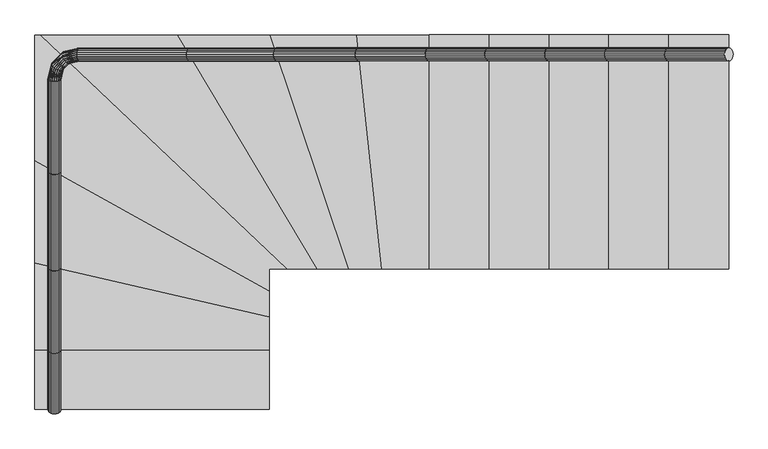
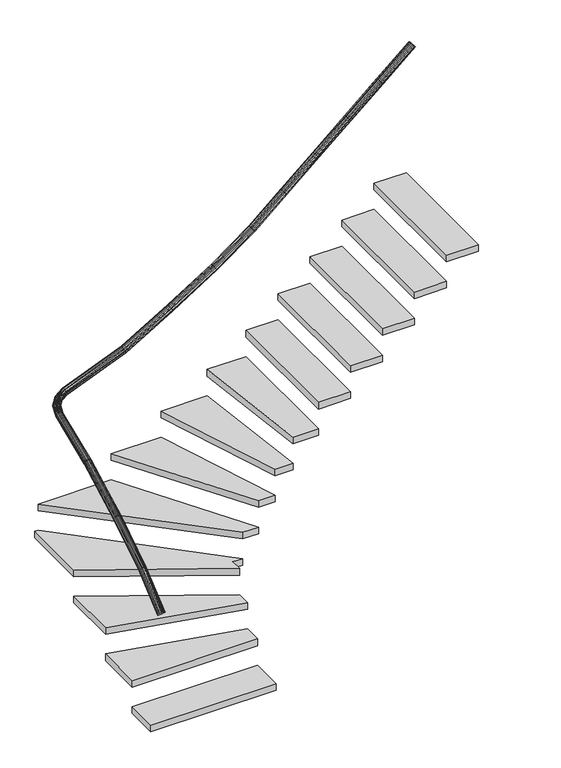
"""IFC4 building model written with IfcOpenShell, lengths in millimetres: stair geometry, 0_3d."""

import ifcopenshell
import ifcopenshell.guid

model = None  # the IFC model being written
_history = None  # IfcOwnerHistory: only IFC2X3 demands one
_inside = {}  # id of a spatial element -> (the spatial element, [elements in it])
_under = {}  # id of a project, library or spatial element -> (it, [spatial elements below it])
_declared = {}  # id of a project -> (the project, [libraries it declares])
_typed = {}  # id of a type object -> (the type object, [elements of that type])
_made_of = {}  # id of a material, layer set ... -> (it, [elements and type objects made of it])


def new_model(schema):
    """Start an empty IFC model of exactly this schema.

    Asked for "IFC4X3", IfcOpenShell would pick the latest addendum, in which some entities
    have other attributes; the version numbers below select the first issue.
    IFC2X3 requires an IfcOwnerHistory on every rooted entity: one is made here for all.
    """
    global model, _history
    if schema == "IFC4X3":
        model = ifcopenshell.file(schema_version=(4, 3, 0, 0))
    else:
        model = ifcopenshell.file(schema=schema)
    _inside.clear()
    _under.clear()
    _declared.clear()
    _typed.clear()
    _made_of.clear()
    _history = None
    if model.schema == "IFC2X3":
        org = make("IfcOrganization", Name="unknown")
        user = make(
            "IfcPersonAndOrganization",
            ThePerson=make("IfcPerson", FamilyName="unknown"),
            TheOrganization=org,
        )
        app = make(
            "IfcApplication",
            ApplicationDeveloper=org,
            Version="unknown",
            ApplicationFullName="unknown",
            ApplicationIdentifier="unknown",
        )
        _history = make(
            "IfcOwnerHistory",
            OwningUser=user,
            OwningApplication=app,
            ChangeAction="ADDED",
            CreationDate=0,
        )
    return model


def make(cls, **values):
    """One entity of the class cls with the attributes given. An attribute that is None is left unset."""
    return model.create_entity(
        cls, **{name: value for name, value in values.items() if value is not None}
    )


def rooted(cls, **values):
    """An entity with a GlobalId (a new one), such as an element, a storey or a relation."""
    return make(cls, GlobalId=ifcopenshell.guid.new(), OwnerHistory=_history, **values)


def si_unit(unit_type, name, prefix=None):
    """IfcSIUnit, for example si_unit("LENGTHUNIT", "METRE", prefix="MILLI")."""
    return make("IfcSIUnit", UnitType=unit_type, Prefix=prefix, Name=name)


def assignment(units):
    """IfcUnitAssignment: the units of a project."""
    return None if units is None else make("IfcUnitAssignment", Units=units)


def point(xyz):
    """IfcCartesianPoint."""
    return None if xyz is None else make("IfcCartesianPoint", Coordinates=xyz)


def direction(xyz):
    """IfcDirection."""
    return None if xyz is None else make("IfcDirection", DirectionRatios=xyz)


def frame(location, z_axis=None, x_axis=None):
    """IfcAxis2Placement3D, a coordinate frame: its origin and axes. An axis left out is left unset."""
    return make(
        "IfcAxis2Placement3D",
        Location=point(location),
        Axis=direction(z_axis),
        RefDirection=direction(x_axis),
    )


def origin():
    """The frame at (0, 0, 0) with its axes left unset."""
    return frame((0.0, 0.0, 0.0))


def origin_with_axes():
    """The frame at (0, 0, 0) with the z axis (0, 0, 1) and the x axis (1, 0, 0) written out."""
    return frame((0.0, 0.0, 0.0), z_axis=(0.0, 0.0, 1.0), x_axis=(1.0, 0.0, 0.0))


def place(relative_to, where):
    """IfcLocalPlacement: puts the frame where relative to a parent placement (None: the world)."""
    return make(
        "IfcLocalPlacement", PlacementRelTo=relative_to, RelativePlacement=where
    )


def context(
    kind, dimensions, precision=None, world=None, true_north=None, identifier=None
):
    """IfcGeometricRepresentationContext, for example the 3D "Model" context."""
    return make(
        "IfcGeometricRepresentationContext",
        ContextIdentifier=identifier,
        ContextType=kind,
        CoordinateSpaceDimension=dimensions,
        Precision=precision,
        WorldCoordinateSystem=world,
        TrueNorth=true_north,
    )


def project(units=None, contexts=None):
    """IfcProject with its units and contexts."""
    return rooted(
        "IfcProject",
        Name="project",
        RepresentationContexts=contexts,
        UnitsInContext=assignment(units),
    )


def spatial(cls, under=None, at=None, **own):
    """A site, building, storey or space (cls), placed at a placement, below another one or the project."""
    s = rooted(cls, ObjectPlacement=at, **own)
    if under is not None:
        _under.setdefault(under.id(), (under, []))[1].append(s)
    return s


def polyline(points):
    """IfcPolyline through the points."""
    return make("IfcPolyline", Points=[point(p) for p in points])


def outline(outer, holes=None, kind="AREA"):
    """IfcArbitraryClosedProfileDef: a profile drawn as a closed curve; with holes, ...WithVoids."""
    if holes is None:
        return make("IfcArbitraryClosedProfileDef", ProfileType=kind, OuterCurve=outer)
    return make(
        "IfcArbitraryProfileDefWithVoids",
        ProfileType=kind,
        OuterCurve=outer,
        InnerCurves=holes,
    )


def extrude(swept, where, along, depth):
    """IfcExtrudedAreaSolid: the profile swept, set in the frame where, extruded along a direction by depth."""
    return make(
        "IfcExtrudedAreaSolid",
        SweptArea=swept,
        Position=where,
        ExtrudedDirection=direction(along),
        Depth=depth,
    )


def faces_of(points, faces, orient=None, outer=None):
    """IfcFace entities. A face is a list of loops; a loop is a list of indices into points, from 0.

    orient and outer hold one flag for each loop. By default every Orientation is true, the
    first loop of a face is its IfcFaceOuterBound and the others are IfcFaceBound.
    """
    made = []
    for i, loops in enumerate(faces):
        bounds = []
        for j, loop in enumerate(loops):
            is_outer = j == 0 if outer is None else outer[i][j]
            bounds.append(
                make(
                    "IfcFaceOuterBound" if is_outer else "IfcFaceBound",
                    Bound=make("IfcPolyLoop", Polygon=[points[k] for k in loop]),
                    Orientation=True if orient is None else orient[i][j],
                )
            )
        made.append(make("IfcFace", Bounds=bounds))
    return made


def faceted_brep(points, faces, orient=None, outer=None, voids=None):
    """IfcFacetedBrep: a solid bounded by flat faces; with voids (closed shells), ...WithVoids."""
    shared = [point(p) for p in points]
    hull = make("IfcClosedShell", CfsFaces=faces_of(shared, faces, orient, outer))
    if voids is None:
        return make("IfcFacetedBrep", Outer=hull)
    return make(
        "IfcFacetedBrepWithVoids",
        Outer=hull,
        Voids=[
            make(cls, CfsFaces=faces_of(shared, fs, o, b)) for cls, fs, o, b in voids
        ],
    )


def shape(context_of_items, identifier, shape_type, items):
    """IfcShapeRepresentation: the items that make up one representation, for example the "Body"."""
    return make(
        "IfcShapeRepresentation",
        ContextOfItems=context_of_items,
        RepresentationIdentifier=identifier,
        RepresentationType=shape_type,
        Items=items,
    )


def source(mapping_origin, context_of_items, identifier, shape_type, items):
    """IfcRepresentationMap: a shape defined once, which mapped items show again and again."""
    return make(
        "IfcRepresentationMap",
        MappingOrigin=mapping_origin,
        MappedRepresentation=shape(context_of_items, identifier, shape_type, items),
    )


def transform(
    local_origin,
    x_axis=None,
    y_axis=None,
    z_axis=None,
    scale=None,
    scale2=None,
    scale3=None,
    uniform=True,
):
    """IfcCartesianTransformationOperator3D, or its non-uniform kind. x_axis, y_axis, z_axis: its Axis1, 2, 3."""
    if uniform:
        return make(
            "IfcCartesianTransformationOperator3D",
            Axis1=direction(x_axis),
            Axis2=direction(y_axis),
            LocalOrigin=point(local_origin),
            Scale=scale,
            Axis3=direction(z_axis),
        )
    return make(
        "IfcCartesianTransformationOperator3DnonUniform",
        Axis1=direction(x_axis),
        Axis2=direction(y_axis),
        LocalOrigin=point(local_origin),
        Scale=scale,
        Axis3=direction(z_axis),
        Scale2=scale2,
        Scale3=scale3,
    )


def mapped(mapping_source, mapping_target):
    """IfcMappedItem: shows the shape of a source again, moved by a transform."""
    return make(
        "IfcMappedItem", MappingSource=mapping_source, MappingTarget=mapping_target
    )


def made_of(thing, what):
    """Note that an element or type object is made of a material, layer set ...; save() writes the relation."""
    if what is not None:
        _made_of.setdefault(what.id(), (what, []))[1].append(thing)
    return thing


def element(
    cls,
    number,
    at=None,
    inside=None,
    cuts=None,
    type_object=None,
    material=None,
    context=None,
    identifier="Body",
    shape_type=None,
    held_by="IfcProductDefinitionShape",
    body=None,
    shapes=None,
    **own,
):
    """One element of the class cls, such as IfcWall. Its Tag is "e" and its number.

    at: its placement. inside: the storey or other place that contains it. cuts: it is an
    opening in that element (IfcRelVoidsElement). A single representation is given by context,
    identifier, shape_type and body (its items); several are given by shapes. held_by: the class
    of the entity that holds the representations. save() writes the other relations.
    """
    e = rooted(cls, Tag="e%d" % number, ObjectPlacement=at, **own)
    if body is not None:
        shapes = [shape(context, identifier, shape_type, body)]
    if shapes is not None:
        e.Representation = make(held_by, Representations=shapes)
    if inside is not None:
        _inside.setdefault(inside.id(), (inside, []))[1].append(e)
    if cuts is not None:
        rooted(
            "IfcRelVoidsElement", RelatingBuildingElement=cuts, RelatedOpeningElement=e
        )
    if type_object is not None:
        _typed.setdefault(type_object.id(), (type_object, []))[1].append(e)
    return made_of(e, material)


def aggregate(whole, parts):
    """IfcRelAggregates: a whole, such as a stair, and the parts it consists of."""
    return rooted("IfcRelAggregates", RelatingObject=whole, RelatedObjects=parts)


def save(model, path):
    """Write the relations noted so far, then the file.

    IfcRelAggregates (storeys below a building ...), IfcRelContainedInSpatialStructure (elements
    in a storey), IfcRelDefinesByType, IfcRelAssociatesMaterial and IfcRelDeclares: one each for
    every whole, place, type object, material and project.
    """
    for whole, parts in _under.values():
        aggregate(whole, parts)
    for where, things in _inside.values():
        rooted(
            "IfcRelContainedInSpatialStructure",
            RelatedElements=things,
            RelatingStructure=where,
        )
    for kind, things in _typed.values():
        rooted("IfcRelDefinesByType", RelatedObjects=things, RelatingType=kind)
    for what, things in _made_of.values():
        rooted("IfcRelAssociatesMaterial", RelatedObjects=things, RelatingMaterial=what)
    for by, libraries in _declared.values():
        rooted("IfcRelDeclares", RelatingContext=by, RelatedDefinitions=libraries)
    model.write(path)


def stair_df875d3e(model_context):
    return source(origin(), model_context, "Body", "SolidModel", [
        extrude(outline(polyline([(0.0, 246.9018591), (0.0, 579.8690495), (900.0, 373.9346688), (900.0, 246.9018591), (0.0, 246.9018591)])), frame((0.0, 0.0, 198.5714286), z_axis=(0.0, 0.0, 1.0), x_axis=(1.0, 0.0, 0.0)), (0.0, 0.0, 1.0), 50.0),
        extrude(outline(polyline([(0.0, 973.1970565), (0.0, 1456.9018591), (22.6704161, 1456.9018591), (970.0, 556.9018591), (900.0, 556.9018591), (900.0, 473.824936), (0.0, 973.1970565)])), frame((0.0, 0.0, 595.7142857), z_axis=(0.0, 0.0, 1.0), x_axis=(1.0, 0.0, 0.0)), (0.0, 0.0, 1.0), 50.0),
        extrude(outline(polyline([(548.8803485, 1456.9018591), (904.7220467, 1456.9018591), (1204.4816265, 556.9018591), (1084.3313864, 556.9018591), (548.8803485, 1456.9018591)])), frame((0.0, 0.0, 992.8571429), z_axis=(0.0, 0.0, 1.0), x_axis=(1.0, 0.0, 0.0)), (0.0, 0.0, 1.0), 50.0),
        faceted_brep([(98.7764129, 251.6675536, 1061.6862641), (100.0, 246.9018591, 1068.1306652), (98.7764129, 242.1361647, 1074.5750662), (95.2254249, 237.8369696, 1080.3886444), (89.6946313, 234.4251091, 1085.0023262), (82.7254249, 232.2345598, 1087.9644922), (75.0, 231.4797479, 1088.985185), (67.2745751, 232.2345598, 1087.9644922), (60.3053687, 234.4251091, 1085.0023262), (54.7745751, 237.8369696, 1080.3886444), (51.2235871, 242.1361647, 1074.5750662), (50.0, 246.9018591, 1068.1306652), (51.2235871, 251.6675536, 1061.6862641), (54.7745751, 255.9667486, 1055.872686), (60.3053687, 259.3786091, 1051.2590042), (67.2745751, 261.5691584, 1048.2968382), (75.0, 262.3239703, 1047.2761453), (82.7254249, 261.5691584, 1048.2968382), (89.6946313, 259.3786091, 1051.2590042), (95.2254249, 255.9667486, 1055.872686), (98.7764129, 558.6819455, 1273.6116568), (100.0, 562.7078511, 1266.7020937), (98.7764129, 566.7337566, 1259.7925307), (95.2254249, 570.3655785, 1253.5593239), (89.6946313, 573.2478087, 1248.6126229), (82.7254249, 575.0983143, 1245.4366454), (75.0, 575.7359551, 1244.3422781), (67.2745751, 575.0983143, 1245.4366454), (60.3053687, 573.2478087, 1248.6126229), (54.7745751, 570.3655785, 1253.5593239), (51.2235871, 566.7337566, 1259.7925307), (50.0, 562.7078511, 1266.7020937), (51.2235871, 558.6819455, 1273.6116568), (54.7745751, 555.0501237, 1279.8448636), (60.3053687, 552.1678935, 1284.7915646), (67.2745751, 550.3173878, 1287.9675421), (75.0, 549.679747, 1289.0619094), (82.7254249, 550.3173878, 1287.9675421), (89.6946313, 552.1678935, 1284.7915646), (95.2254249, 555.0501237, 1279.8448636)], [[[0, 1, 2, 3, 4, 5, 6, 7, 8, 9, 10, 11, 12, 13, 14, 15, 16, 17, 18, 19]], [[20, 21, 22, 23, 24, 25, 26, 27, 28, 29, 30, 31, 32, 33, 34, 35, 36, 37, 38, 39]], [[2, 1, 21, 20]], [[3, 2, 20, 39]], [[4, 3, 39, 38]], [[5, 4, 38, 37]], [[6, 5, 37, 36]], [[7, 6, 36, 35]], [[8, 7, 35, 34]], [[9, 8, 34, 33]], [[10, 9, 33, 32]], [[11, 10, 32, 31]], [[12, 11, 31, 30]], [[13, 12, 30, 29]], [[14, 13, 29, 28]], [[15, 14, 28, 27]], [[16, 15, 27, 26]], [[17, 16, 26, 25]], [[18, 17, 25, 24]], [[19, 18, 24, 23]], [[0, 19, 23, 22]], [[1, 0, 22, 21]]]),
        extrude(outline(polyline([(1974.6018366, 1456.9018591), (2204.6018366, 1456.9018591), (2204.6018366, 556.9018591), (1974.6018366, 556.9018591), (1974.6018366, 1456.9018591)])), frame((0.0, 0.0, 1985.7142857), z_axis=(0.0, 0.0, 1.0), x_axis=(1.0, 0.0, 0.0)), (0.0, 0.0, 1.0), 50.0),
        extrude(outline(polyline([(1.2235871, -7.9923214), (0.0, 0.0), (1.2235871, 7.9923214), (4.7745752, 15.2022986), (10.3053687, 20.9241691), (17.2745752, 24.5978359), (25.0, 25.8636953), (32.7254249, 24.5978359), (39.6946313, 20.9241691), (45.2254249, 15.2022986), (48.7764129, 7.9923214), (50.0, 0.0), (48.7764129, -7.9923214), (45.2254249, -15.2022986), (39.6946313, -20.9241691), (32.7254249, -24.5978359), (25.0, -25.8636953), (17.2745752, -24.5978359), (10.3053687, -20.9241691), (4.7745752, -15.2022986), (1.2235871, -7.9923214)])), frame((2204.6018366, 1356.9018591, 3053.8449509), z_axis=(0.7569287102857765, 0.0, 0.6534974579484691), x_axis=(0.0, 1.0, 0.0)), (0.0, 0.0, 1.0), 303.8595272),
        faceted_brep([(98.7764129, 566.7337566, 1259.7925307), (100.0, 562.7078511, 1266.7020937), (98.7764129, 558.6819455, 1273.6116568), (95.2254249, 555.0501237, 1279.8448636), (89.6946313, 552.1678935, 1284.7915646), (82.7254249, 550.3173878, 1287.9675421), (75.0, 549.679747, 1289.0619094), (67.2745751, 550.3173878, 1287.9675421), (60.3053687, 552.1678935, 1284.7915646), (54.7745751, 555.0501237, 1279.8448636), (51.2235871, 558.6819455, 1273.6116568), (50.0, 562.7078511, 1266.7020937), (51.2235871, 566.7337566, 1259.7925307), (54.7745751, 570.3655785, 1253.5593239), (60.3053687, 573.2478087, 1248.6126229), (67.2745751, 575.0983143, 1245.4366454), (75.0, 575.7359551, 1244.3422781), (82.7254249, 575.0983143, 1245.4366454), (89.6946313, 573.2478087, 1248.6126229), (95.2254249, 570.3655785, 1253.5593239), (98.7764129, 928.1440687, 1472.4992177), (100.0, 931.5827131, 1465.2735223), (98.7764129, 935.0213576, 1458.0478269), (95.2254249, 938.1234035, 1451.529433), (89.6946313, 940.5852011, 1446.3564062), (82.7254249, 942.1657724, 1443.0351186), (75.0, 942.7104002, 1441.8906809), (67.2745751, 942.1657724, 1443.0351186), (60.3053687, 940.5852011, 1446.3564062), (54.7745751, 938.1234035, 1451.529433), (51.2235871, 935.0213576, 1458.0478269), (50.0, 931.5827131, 1465.2735223), (51.2235871, 928.1440687, 1472.4992177), (54.7745751, 925.0420228, 1479.0176117), (60.3053687, 922.5802252, 1484.1906384), (67.2745751, 920.9996538, 1487.511926), (75.0, 920.4550261, 1488.6563638), (82.7254249, 920.9996538, 1487.511926), (89.6946313, 922.5802252, 1484.1906384), (95.2254249, 925.0420228, 1479.0176117)], [[[0, 1, 2, 3, 4, 5, 6, 7, 8, 9, 10, 11, 12, 13, 14, 15, 16, 17, 18, 19]], [[20, 21, 22, 23, 24, 25, 26, 27, 28, 29, 30, 31, 32, 33, 34, 35, 36, 37, 38, 39]], [[2, 1, 21, 20]], [[3, 2, 20, 39]], [[4, 3, 39, 38]], [[5, 4, 38, 37]], [[6, 5, 37, 36]], [[7, 6, 36, 35]], [[8, 7, 35, 34]], [[9, 8, 34, 33]], [[10, 9, 33, 32]], [[11, 10, 32, 31]], [[12, 11, 31, 30]], [[13, 12, 30, 29]], [[14, 13, 29, 28]], [[15, 14, 28, 27]], [[16, 15, 27, 26]], [[17, 16, 26, 25]], [[18, 17, 25, 24]], [[19, 18, 24, 23]], [[0, 19, 23, 22]], [[1, 0, 22, 21]]]),
        extrude(outline(polyline([(2434.6018366, 1456.9018591), (2664.6018366, 1456.9018591), (2664.6018366, 556.9018591), (2434.6018366, 556.9018591), (2434.6018366, 1456.9018591)])), frame((0.0, 0.0, 2382.8571429), z_axis=(0.0, 0.0, 1.0), x_axis=(1.0, 0.0, 0.0)), (0.0, 0.0, 1.0), 50.0),
        faceted_brep([(98.7764129, 935.0213576, 1458.0478269), (100.0, 931.5827131, 1465.2735223), (98.7764129, 928.1440687, 1472.4992177), (95.2254249, 925.0420228, 1479.0176117), (89.6946313, 922.5802252, 1484.1906384), (82.7254249, 920.9996538, 1487.511926), (75.0, 920.4550261, 1488.6563638), (67.2745751, 920.9996538, 1487.511926), (60.3053687, 922.5802252, 1484.1906384), (54.7745751, 925.0420228, 1479.0176117), (51.2235871, 928.1440687, 1472.4992177), (50.0, 931.5827131, 1465.2735223), (51.2235871, 935.0213576, 1458.0478269), (54.7745751, 938.1234035, 1451.529433), (60.3053687, 940.5852011, 1446.3564062), (67.2745751, 942.1657724, 1443.0351186), (75.0, 942.7104002, 1441.8906809), (82.7254249, 942.1657724, 1443.0351186), (89.6946313, 940.5852011, 1446.3564062), (95.2254249, 938.1234035, 1451.529433), (98.7764129, 1283.3224302, 1620.3777918), (100.0, 1286.3944101, 1612.9994356), (98.7764129, 1289.46639, 1605.6210794), (95.2254249, 1292.2376632, 1598.9649681), (89.6946313, 1294.436958, 1593.6826483), (82.7254249, 1295.8489921, 1590.2911902), (75.0, 1296.335546, 1589.1225734), (67.2745751, 1295.8489921, 1590.2911902), (60.3053687, 1294.436958, 1593.6826483), (54.7745751, 1292.2376632, 1598.9649681), (51.2235871, 1289.46639, 1605.6210794), (50.0, 1286.3944101, 1612.9994356), (51.2235871, 1283.3224302, 1620.3777918), (54.7745751, 1280.5511571, 1627.0339031), (60.3053687, 1278.3518623, 1632.3162229), (67.2745751, 1276.9398281, 1635.707681), (75.0, 1276.4532743, 1636.8762979), (82.7254249, 1276.9398281, 1635.707681), (89.6946313, 1278.3518623, 1632.3162229), (95.2254249, 1280.5511571, 1627.0339031)], [[[0, 1, 2, 3, 4, 5, 6, 7, 8, 9, 10, 11, 12, 13, 14, 15, 16, 17, 18, 19]], [[20, 21, 22, 23, 24, 25, 26, 27, 28, 29, 30, 31, 32, 33, 34, 35, 36, 37, 38, 39]], [[2, 1, 21, 20]], [[3, 2, 20, 39]], [[4, 3, 39, 38]], [[5, 4, 38, 37]], [[6, 5, 37, 36]], [[7, 6, 36, 35]], [[8, 7, 35, 34]], [[9, 8, 34, 33]], [[10, 9, 33, 32]], [[11, 10, 32, 31]], [[12, 11, 31, 30]], [[13, 12, 30, 29]], [[14, 13, 29, 28]], [[15, 14, 28, 27]], [[16, 15, 27, 26]], [[17, 16, 26, 25]], [[18, 17, 25, 24]], [[19, 18, 24, 23]], [[0, 19, 23, 22]], [[1, 0, 22, 21]]]),
        faceted_brep([(1249.3489942, 1358.1254462, 2252.9513864), (1244.8437697, 1356.9018591, 2259.5592366), (1240.3385453, 1358.1254462, 2266.1670868), (1236.2743236, 1361.6764343, 2272.1281145), (1233.048939, 1367.2072278, 2276.858813), (1230.9781146, 1374.1764343, 2279.8961083), (1230.2645572, 1381.9018591, 2280.942689), (1230.9781146, 1389.627284, 2279.8961083), (1233.048939, 1396.5964904, 2276.858813), (1236.2743236, 1402.127284, 2272.1281145), (1240.3385453, 1405.678272, 2266.1670868), (1244.8437697, 1406.9018591, 2259.5592366), (1249.3489942, 1405.678272, 2252.9513864), (1253.4132159, 1402.127284, 2246.9903587), (1256.6386004, 1396.5964904, 2242.2596602), (1258.7094248, 1389.627284, 2239.2223649), (1259.4229823, 1381.9018591, 2238.1757842), (1258.7094248, 1374.1764343, 2239.2223649), (1256.6386004, 1367.2072278, 2242.2596602), (1253.4132159, 1361.6764343, 2246.9903587), (1509.6138519, 1358.1254462, 2464.383151), (1514.6018366, 1356.9018591, 2458.1306652), (1519.5898213, 1358.1254462, 2451.8781793), (1524.0895473, 1361.6764343, 2446.2377304), (1527.6605501, 1367.2072278, 2441.7614447), (1529.9532751, 1374.1764343, 2438.8874925), (1530.7432942, 1381.9018591, 2437.897196), (1529.9532751, 1389.627284, 2438.8874925), (1527.6605501, 1396.5964904, 2441.7614447), (1524.0895473, 1402.127284, 2446.2377304), (1519.5898213, 1405.678272, 2451.8781793), (1514.6018366, 1406.9018591, 2458.1306652), (1509.6138519, 1405.678272, 2464.383151), (1505.1141259, 1402.127284, 2470.0236), (1501.5431231, 1396.5964904, 2474.4998856), (1499.2503981, 1389.627284, 2477.3738379), (1498.460379, 1381.9018591, 2478.3641344), (1499.2503981, 1374.1764343, 2477.3738379), (1501.5431231, 1367.2072278, 2474.4998856), (1505.1141259, 1361.6764343, 2470.0236)], [[[0, 1, 2, 3, 4, 5, 6, 7, 8, 9, 10, 11, 12, 13, 14, 15, 16, 17, 18, 19]], [[20, 21, 22, 23, 24, 25, 26, 27, 28, 29, 30, 31, 32, 33, 34, 35, 36, 37, 38, 39]], [[2, 1, 21, 20]], [[3, 2, 20, 39]], [[4, 3, 39, 38]], [[5, 4, 38, 37]], [[6, 5, 37, 36]], [[7, 6, 36, 35]], [[8, 7, 35, 34]], [[9, 8, 34, 33]], [[10, 9, 33, 32]], [[11, 10, 32, 31]], [[12, 11, 31, 30]], [[13, 12, 30, 29]], [[14, 13, 29, 28]], [[15, 14, 28, 27]], [[16, 15, 27, 26]], [[17, 16, 26, 25]], [[18, 17, 25, 24]], [[19, 18, 24, 23]], [[0, 19, 23, 22]], [[1, 0, 22, 21]]]),
        extrude(outline(polyline([(1.2235871, -7.9923214), (0.0, 0.0), (1.2235871, 7.9923214), (4.7745752, 15.2022986), (10.3053687, 20.924169), (17.2745752, 24.5978359), (25.0, 25.8636953), (32.7254249, 24.5978359), (39.6946313, 20.924169), (45.2254249, 15.2022986), (48.7764129, 7.9923214), (50.0, 0.0), (48.7764129, -7.9923214), (45.2254249, -15.2022986), (39.6946313, -20.9241691), (32.7254249, -24.597836), (25.0, -25.8636953), (17.2745752, -24.597836), (10.3053687, -20.9241691), (4.7745752, -15.2022986), (1.2235871, -7.9923214)])), frame((2434.6018366, 1356.9018591, 3252.4163795), z_axis=(0.7569287102857786, 0.0, 0.6534974579484667), x_axis=(0.0, 1.0, 0.0)), (0.0, 0.0, 1.0), 303.8595272),
        extrude(outline(polyline([(0.0, 579.8690495), (0.0, 973.1970565), (900.0, 473.824936), (900.0, 373.9346688), (0.0, 579.8690495)])), frame((0.0, 0.0, 397.1428571), z_axis=(0.0, 0.0, 1.0), x_axis=(1.0, 0.0, 0.0)), (0.0, 0.0, 1.0), 50.0),
        extrude(outline(polyline([(22.6704161, 1456.9018591), (548.8803485, 1456.9018591), (1084.3313864, 556.9018591), (970.0, 556.9018591), (22.6704161, 1456.9018591)])), frame((0.0, 0.0, 794.2857143), z_axis=(0.0, 0.0, 1.0), x_axis=(1.0, 0.0, 0.0)), (0.0, 0.0, 1.0), 50.0),
        extrude(outline(polyline([(1.2235871, -7.9923214), (0.0, 0.0), (1.2235871, 7.9923214), (4.7745752, 15.2022987), (10.3053687, 20.9241691), (17.2745752, 24.597836), (25.0, 25.8636953), (32.7254249, 24.597836), (39.6946313, 20.9241691), (45.2254249, 15.2022987), (48.7764129, 7.9923214), (50.0, 0.0), (48.7764129, -7.9923214), (45.2254249, -15.2022986), (39.6946313, -20.924169), (32.7254249, -24.5978359), (25.0, -25.8636953), (17.2745752, -24.5978359), (10.3053687, -20.924169), (4.7745752, -15.2022986), (1.2235871, -7.9923214)])), frame((1744.6018366, 1356.9018591, 2656.7020937), z_axis=(0.7569287102857375, 0.0, 0.6534974579485143), x_axis=(0.0, 1.0, 0.0)), (0.0, 0.0, 1.0), 303.8595272),
        faceted_brep([(933.8654844, 1358.1254462, 2054.1646194), (929.7020117, 1356.9018591, 2060.987808), (925.538539, 1358.1254462, 2067.8109967), (921.782616, 1361.6764343, 2073.966284), (918.8018987, 1367.2072278, 2078.8511477), (916.8881603, 1374.1764343, 2081.9874233), (916.228731, 1381.9018591, 2083.0681102), (916.8881603, 1389.627284, 2081.9874233), (918.8018987, 1396.5964904, 2078.8511477), (921.782616, 1402.127284, 2073.966284), (925.538539, 1405.678272, 2067.8109967), (929.7020117, 1406.9018591, 2060.987808), (933.8654844, 1405.678272, 2054.1646194), (937.6214074, 1402.127284, 2048.009332), (940.6021247, 1396.5964904, 2043.1244683), (942.515863, 1389.627284, 2039.9881928), (943.1752923, 1381.9018591, 2038.9075058), (942.515863, 1374.1764343, 2039.9881928), (940.6021247, 1367.2072278, 2043.1244683), (937.6214074, 1361.6764343, 2048.009332), (1240.3385453, 1358.1254462, 2266.1670868), (1244.8437697, 1356.9018591, 2259.5592366), (1249.3489942, 1358.1254462, 2252.9513864), (1253.4132159, 1361.6764343, 2246.9903587), (1256.6386004, 1367.2072278, 2242.2596602), (1258.7094248, 1374.1764343, 2239.2223649), (1259.4229823, 1381.9018591, 2238.1757842), (1258.7094248, 1389.627284, 2239.2223649), (1256.6386004, 1396.5964904, 2242.2596602), (1253.4132159, 1402.127284, 2246.9903587), (1249.3489942, 1405.678272, 2252.9513864), (1244.8437697, 1406.9018591, 2259.5592366), (1240.3385453, 1405.678272, 2266.1670868), (1236.2743236, 1402.127284, 2272.1281145), (1233.048939, 1396.5964904, 2276.858813), (1230.9781146, 1389.627284, 2279.8961083), (1230.2645572, 1381.9018591, 2280.942689), (1230.9781146, 1374.1764343, 2279.8961083), (1233.048939, 1367.2072278, 2276.858813), (1236.2743236, 1361.6764343, 2272.1281145)], [[[0, 1, 2, 3, 4, 5, 6, 7, 8, 9, 10, 11, 12, 13, 14, 15, 16, 17, 18, 19]], [[20, 21, 22, 23, 24, 25, 26, 27, 28, 29, 30, 31, 32, 33, 34, 35, 36, 37, 38, 39]], [[2, 1, 21, 20]], [[3, 2, 20, 39]], [[4, 3, 39, 38]], [[5, 4, 38, 37]], [[6, 5, 37, 36]], [[7, 6, 36, 35]], [[8, 7, 35, 34]], [[9, 8, 34, 33]], [[10, 9, 33, 32]], [[11, 10, 32, 31]], [[12, 11, 31, 30]], [[13, 12, 30, 29]], [[14, 13, 29, 28]], [[15, 14, 28, 27]], [[16, 15, 27, 26]], [[17, 16, 26, 25]], [[18, 17, 25, 24]], [[19, 18, 24, 23]], [[0, 19, 23, 22]], [[1, 0, 22, 21]]]),
        faceted_brep([(597.0493296, 1358.1254462, 1855.2297082), (593.5012683, 1356.9018591, 1862.4163795), (589.9532071, 1358.1254462, 1869.6030507), (586.7524548, 1361.6764343, 1876.0862405), (584.2123234, 1367.2072278, 1881.231329), (582.5814586, 1374.1764343, 1884.5346792), (582.019501, 1381.9018591, 1885.6729361), (582.5814586, 1389.627284, 1884.5346792), (584.2123234, 1396.5964904, 1881.231329), (586.7524548, 1402.127284, 1876.0862405), (589.9532071, 1405.678272, 1869.6030507), (593.5012683, 1406.9018591, 1862.4163795), (597.0493296, 1405.678272, 1855.2297082), (600.2500819, 1402.127284, 1848.7465184), (602.7902133, 1396.5964904, 1843.6014299), (604.421078, 1389.627284, 1840.2980797), (604.9830357, 1381.9018591, 1839.1598228), (604.421078, 1374.1764343, 1840.2980797), (602.7902133, 1367.2072278, 1843.6014299), (600.2500819, 1361.6764343, 1848.7465184), (925.538539, 1358.1254462, 2067.8109967), (929.7020117, 1356.9018591, 2060.987808), (933.8654844, 1358.1254462, 2054.1646194), (937.6214074, 1361.6764343, 2048.009332), (940.6021247, 1367.2072278, 2043.1244683), (942.515863, 1374.1764343, 2039.9881928), (943.1752923, 1381.9018591, 2038.9075058), (942.515863, 1389.627284, 2039.9881928), (940.6021247, 1396.5964904, 2043.1244683), (937.6214074, 1402.127284, 2048.009332), (933.8654844, 1405.678272, 2054.1646194), (929.7020117, 1406.9018591, 2060.987808), (925.538539, 1405.678272, 2067.8109967), (921.782616, 1402.127284, 2073.966284), (918.8018987, 1396.5964904, 2078.8511477), (916.8881603, 1389.627284, 2081.9874233), (916.228731, 1381.9018591, 2083.0681102), (916.8881603, 1374.1764343, 2081.9874233), (918.8018987, 1367.2072278, 2078.8511477), (921.782616, 1361.6764343, 2073.966284)], [[[0, 1, 2, 3, 4, 5, 6, 7, 8, 9, 10, 11, 12, 13, 14, 15, 16, 17, 18, 19]], [[20, 21, 22, 23, 24, 25, 26, 27, 28, 29, 30, 31, 32, 33, 34, 35, 36, 37, 38, 39]], [[2, 1, 21, 20]], [[3, 2, 20, 39]], [[4, 3, 39, 38]], [[5, 4, 38, 37]], [[6, 5, 37, 36]], [[7, 6, 36, 35]], [[8, 7, 35, 34]], [[9, 8, 34, 33]], [[10, 9, 33, 32]], [[11, 10, 32, 31]], [[12, 11, 31, 30]], [[13, 12, 30, 29]], [[14, 13, 29, 28]], [[15, 14, 28, 27]], [[16, 15, 27, 26]], [[17, 16, 26, 25]], [[18, 17, 25, 24]], [[19, 18, 24, 23]], [[0, 19, 23, 22]], [[1, 0, 22, 21]]]),
        faceted_brep([(98.7764129, 1289.46639, 1605.6210794), (100.0, 1286.3944101, 1612.9994356), (98.7764129, 1283.3224302, 1620.3777918), (95.2254249, 1280.5511571, 1627.0339031), (89.6946313, 1278.3518623, 1632.3162229), (82.7254249, 1276.9398281, 1635.707681), (75.0, 1276.4532743, 1636.8762979), (67.2745751, 1276.9398281, 1635.707681), (60.3053687, 1278.3518623, 1632.3162229), (54.7745751, 1280.5511571, 1627.0339031), (51.2235871, 1283.3224302, 1620.3777918), (50.0, 1286.3944101, 1612.9994356), (51.2235871, 1289.46639, 1605.6210794), (54.7745751, 1292.2376632, 1598.9649681), (60.3053687, 1294.436958, 1593.6826483), (67.2745751, 1295.8489921, 1590.2911902), (75.0, 1296.335546, 1589.1225734), (82.7254249, 1295.8489921, 1590.2911902), (89.6946313, 1294.436958, 1593.6826483), (95.2254249, 1292.2376632, 1598.9649681), (108.8679012, 1324.8479302, 1638.9123688), (105.9144976, 1321.9997167, 1645.879395), (101.1034244, 1320.6050585, 1652.1644401), (94.9056231, 1320.8004745, 1657.1522801), (87.9277774, 1322.5668359, 1660.3546705), (80.8529277, 1325.7312391, 1661.4581391), (74.3736094, 1329.9839302, 1660.3546705), (69.1240635, 1334.9086261, 1657.1522801), (65.6181519, 1340.0232633, 1652.1644401), (64.1990579, 1344.8271855, 1645.879395), (65.0056921, 1348.8501513, 1638.9123688), (67.9590957, 1351.6983647, 1631.9453426), (72.7701688, 1353.0930229, 1625.6602975), (78.9679702, 1352.8976069, 1620.6724574), (85.9458159, 1351.1312455, 1617.470067), (93.0206656, 1347.9668423, 1616.3665985), (99.4999839, 1343.7141513, 1617.470067), (104.7495298, 1338.7894554, 1620.6724574), (108.2554414, 1333.6748181, 1625.6602975), (109.6745354, 1328.870896, 1631.9453426), (132.1170605, 1348.0291684, 1666.2859781), (128.1175831, 1347.2454175, 1673.2691208), (123.3397137, 1348.6878091, 1679.5687049), (118.2511434, 1352.215152, 1684.5680831), (113.3499769, 1357.4821652, 1687.7778814), (109.1159746, 1363.9732768, 1688.8839026), (105.96359, 1371.0530916, 1687.7778814), (104.2014005, 1378.028588, 1684.5680831), (104.0019016, 1384.2169558, 1679.5687049), (105.3846216, 1389.0124344, 1673.2691208), (108.2142101, 1391.9456089, 1666.2859781), (112.2136875, 1392.7293599, 1659.3028354), (116.9915569, 1391.2869683, 1653.0032514), (122.0801271, 1387.7596254, 1648.0038732), (126.9812936, 1382.4926122, 1644.7940748), (131.215296, 1376.0015006, 1643.6880537), (134.3676806, 1368.9216857, 1644.7940748), (136.1298701, 1361.9461894, 1648.0038732), (136.329369, 1355.7578216, 1653.0032514), (134.946649, 1350.962343, 1659.3028354), (170.8141891, 1356.9018591, 1691.7803901), (167.8223333, 1358.1254462, 1699.1915978), (165.1233413, 1361.6764343, 1705.8773449), (162.981409, 1367.2072278, 1711.1831838), (161.6062039, 1374.1764343, 1714.5897421), (161.1323405, 1381.9018591, 1715.7635621), (161.6062039, 1389.627284, 1714.5897421), (162.981409, 1396.5964904, 1711.1831838), (165.1233413, 1402.127284, 1705.8773449), (167.8223333, 1405.678272, 1699.1915978), (170.8141891, 1406.9018591, 1691.7803901), (173.8060448, 1405.678272, 1684.3691823), (176.5050369, 1402.127284, 1677.6834352), (178.6469691, 1396.5964904, 1672.3775963), (180.0221742, 1389.627284, 1668.971038), (180.4960376, 1381.9018591, 1667.797218), (180.0221742, 1374.1764343, 1668.971038), (178.6469691, 1367.2072278, 1672.3775963), (176.5050369, 1361.6764343, 1677.6834352), (173.8060448, 1358.1254462, 1684.3691823), (589.9532071, 1358.1254462, 1869.6030507), (593.5012683, 1356.9018591, 1862.4163795), (597.0493296, 1358.1254462, 1855.2297082), (600.2500819, 1361.6764343, 1848.7465184), (602.7902133, 1367.2072278, 1843.6014299), (604.421078, 1374.1764343, 1840.2980797), (604.9830357, 1381.9018591, 1839.1598228), (604.421078, 1389.627284, 1840.2980797), (602.7902133, 1396.5964904, 1843.6014299), (600.2500819, 1402.127284, 1848.7465184), (597.0493296, 1405.678272, 1855.2297082), (593.5012683, 1406.9018591, 1862.4163795), (589.9532071, 1405.678272, 1869.6030507), (586.7524548, 1402.127284, 1876.0862405), (584.2123234, 1396.5964904, 1881.231329), (582.5814586, 1389.627284, 1884.5346792), (582.019501, 1381.9018591, 1885.6729361), (582.5814586, 1374.1764343, 1884.5346792), (584.2123234, 1367.2072278, 1881.231329), (586.7524548, 1361.6764343, 1876.0862405)], [[[0, 1, 2, 3, 4, 5, 6, 7, 8, 9, 10, 11, 12, 13, 14, 15, 16, 17, 18, 19]], [[2, 1, 20]], [[21, 2, 20]], [[3, 2, 21]], [[22, 3, 21]], [[4, 3, 22]], [[23, 4, 22]], [[5, 4, 23]], [[24, 5, 23]], [[6, 5, 24]], [[25, 6, 24]], [[7, 6, 25]], [[26, 7, 25]], [[8, 7, 26]], [[27, 8, 26]], [[9, 8, 27]], [[28, 9, 27]], [[10, 9, 28]], [[29, 10, 28]], [[11, 10, 29]], [[30, 11, 29]], [[12, 11, 30]], [[31, 12, 30]], [[13, 12, 31]], [[32, 13, 31]], [[14, 13, 32]], [[33, 14, 32]], [[15, 14, 33]], [[34, 15, 33]], [[16, 15, 34]], [[35, 16, 34]], [[17, 16, 35]], [[36, 17, 35]], [[18, 17, 36]], [[37, 18, 36]], [[19, 18, 37]], [[38, 19, 37]], [[0, 19, 38]], [[39, 0, 38]], [[1, 0, 39]], [[20, 1, 39]], [[21, 20, 40]], [[41, 21, 40]], [[22, 21, 41]], [[42, 22, 41]], [[23, 22, 42]], [[43, 23, 42]], [[24, 23, 43]], [[44, 24, 43]], [[25, 24, 44]], [[45, 25, 44]], [[26, 25, 45]], [[46, 26, 45]], [[27, 26, 46]], [[47, 27, 46]], [[28, 27, 47]], [[48, 28, 47]], [[29, 28, 48]], [[49, 29, 48]], [[30, 29, 49]], [[50, 30, 49]], [[31, 30, 50]], [[51, 31, 50]], [[32, 31, 51]], [[52, 32, 51]], [[33, 32, 52]], [[53, 33, 52]], [[34, 33, 53]], [[54, 34, 53]], [[35, 34, 54]], [[55, 35, 54]], [[36, 35, 55]], [[56, 36, 55]], [[37, 36, 56]], [[57, 37, 56]], [[38, 37, 57]], [[58, 38, 57]], [[39, 38, 58]], [[59, 39, 58]], [[20, 39, 59]], [[40, 20, 59]], [[41, 40, 60]], [[61, 41, 60]], [[42, 41, 61]], [[62, 42, 61]], [[43, 42, 62]], [[63, 43, 62]], [[44, 43, 63]], [[64, 44, 63]], [[45, 44, 64]], [[65, 45, 64]], [[46, 45, 65]], [[66, 46, 65]], [[47, 46, 66]], [[67, 47, 66]], [[48, 47, 67]], [[68, 48, 67]], [[49, 48, 68]], [[69, 49, 68]], [[50, 49, 69]], [[70, 50, 69]], [[51, 50, 70]], [[71, 51, 70]], [[52, 51, 71]], [[72, 52, 71]], [[53, 52, 72]], [[73, 53, 72]], [[54, 53, 73]], [[74, 54, 73]], [[55, 54, 74]], [[75, 55, 74]], [[56, 55, 75]], [[76, 56, 75]], [[57, 56, 76]], [[77, 57, 76]], [[58, 57, 77]], [[78, 58, 77]], [[59, 58, 78]], [[79, 59, 78]], [[40, 59, 79]], [[60, 40, 79]], [[80, 81, 82, 83, 84, 85, 86, 87, 88, 89, 90, 91, 92, 93, 94, 95, 96, 97, 98, 99]], [[61, 60, 81, 80]], [[62, 61, 80, 99]], [[63, 62, 99, 98]], [[64, 63, 98, 97]], [[65, 64, 97, 96]], [[66, 65, 96, 95]], [[67, 66, 95, 94]], [[68, 67, 94, 93]], [[69, 68, 93, 92]], [[70, 69, 92, 91]], [[71, 70, 91, 90]], [[72, 71, 90, 89]], [[73, 72, 89, 88]], [[74, 73, 88, 87]], [[75, 74, 87, 86]], [[76, 75, 86, 85]], [[77, 76, 85, 84]], [[78, 77, 84, 83]], [[79, 78, 83, 82]], [[60, 79, 82, 81]]]),
        extrude(outline(polyline([(1.2235871, -7.9923214), (0.0, 0.0), (1.2235871, 7.9923214), (4.7745752, 15.2022986), (10.3053687, 20.9241691), (17.2745752, 24.5978359), (25.0, 25.8636953), (32.7254249, 24.5978359), (39.6946313, 20.9241691), (45.2254249, 15.2022986), (48.7764129, 7.9923214), (50.0, 0.0), (48.7764129, -7.9923214), (45.2254249, -15.2022986), (39.6946313, -20.924169), (32.7254249, -24.5978359), (25.0, -25.8636953), (17.2745752, -24.5978359), (10.3053687, -20.924169), (4.7745752, -15.2022986), (1.2235871, -7.9923214)])), frame((1974.6018366, 1356.9018591, 2855.2735223), z_axis=(0.7569287102857345, 0.0, 0.6534974579485179), x_axis=(0.0, 1.0, 0.0)), (0.0, 0.0, 1.0), 303.8595272),
        extrude(outline(polyline([(0.0, 16.9018591), (0.0, 246.9018591), (900.0, 246.9018591), (900.0, 16.9018591), (0.0, 16.9018591)])), origin_with_axes(), (0.0, 0.0, 1.0), 50.0),
        extrude(outline(polyline([(1744.6018366, 1456.9018591), (1974.6018366, 1456.9018591), (1974.6018366, 556.9018591), (1744.6018366, 556.9018591), (1744.6018366, 1456.9018591)])), frame((0.0, 0.0, 1787.1428571), z_axis=(0.0, 0.0, 1.0), x_axis=(1.0, 0.0, 0.0)), (0.0, 0.0, 1.0), 50.0),
        faceted_brep([(98.7764129, 22.1248208, 863.5096191), (100.0, 16.9018591, 869.5592366), (98.7764129, 11.6788974, 875.6088541), (95.2254249, 6.9671956, 881.0662929), (89.6946313, 3.2279679, 885.3973409), (82.7254249, 0.8272359, 888.1780448), (75.0, 0.0, 889.1362101), (67.2745751, 0.8272359, 888.1780448), (60.3053687, 3.2279679, 885.3973409), (54.7745751, 6.9671956, 881.0662929), (51.2235871, 11.6788974, 875.6088541), (50.0, 16.9018591, 869.5592366), (51.2235871, 22.1248208, 863.5096191), (54.7745751, 26.8365226, 858.0521803), (60.3053687, 30.5757504, 853.7211323), (67.2745751, 32.9764824, 850.9404284), (75.0, 33.8037182, 849.9822631), (82.7254249, 32.9764824, 850.9404284), (89.6946313, 30.5757504, 853.7211323), (95.2254249, 26.8365226, 858.0521803), (98.7764129, 242.1361647, 1074.5750662), (100.0, 246.9018591, 1068.1306652), (98.7764129, 251.6675536, 1061.6862641), (95.2254249, 255.9667486, 1055.872686), (89.6946313, 259.3786091, 1051.2590042), (82.7254249, 261.5691584, 1048.2968382), (75.0, 262.3239703, 1047.2761453), (67.2745751, 261.5691584, 1048.2968382), (60.3053687, 259.3786091, 1051.2590042), (54.7745751, 255.9667486, 1055.872686), (51.2235871, 251.6675536, 1061.6862641), (50.0, 246.9018591, 1068.1306652), (51.2235871, 242.1361647, 1074.5750662), (54.7745751, 237.8369696, 1080.3886444), (60.3053687, 234.4251091, 1085.0023262), (67.2745751, 232.2345598, 1087.9644922), (75.0, 231.4797479, 1088.985185), (82.7254249, 232.2345598, 1087.9644922), (89.6946313, 234.4251091, 1085.0023262), (95.2254249, 237.8369696, 1080.3886444)], [[[0, 1, 2, 3, 4, 5, 6, 7, 8, 9, 10, 11, 12, 13, 14, 15, 16, 17, 18, 19]], [[20, 21, 22, 23, 24, 25, 26, 27, 28, 29, 30, 31, 32, 33, 34, 35, 36, 37, 38, 39]], [[2, 1, 21, 20]], [[3, 2, 20, 39]], [[4, 3, 39, 38]], [[5, 4, 38, 37]], [[6, 5, 37, 36]], [[7, 6, 36, 35]], [[8, 7, 35, 34]], [[9, 8, 34, 33]], [[10, 9, 33, 32]], [[11, 10, 32, 31]], [[12, 11, 31, 30]], [[13, 12, 30, 29]], [[14, 13, 29, 28]], [[15, 14, 28, 27]], [[16, 15, 27, 26]], [[17, 16, 26, 25]], [[18, 17, 25, 24]], [[19, 18, 24, 23]], [[0, 19, 23, 22]], [[1, 0, 22, 21]]]),
        extrude(outline(polyline([(2204.6018366, 1456.9018591), (2434.6018366, 1456.9018591), (2434.6018366, 556.9018591), (2204.6018366, 556.9018591), (2204.6018366, 1456.9018591)])), frame((0.0, 0.0, 2184.2857143), z_axis=(0.0, 0.0, 1.0), x_axis=(1.0, 0.0, 0.0)), (0.0, 0.0, 1.0), 50.0),
        extrude(outline(polyline([(1514.6018366, 1456.9018591), (1744.6018366, 1456.9018591), (1744.6018366, 556.9018591), (1514.6018366, 556.9018591), (1514.6018366, 1456.9018591)])), frame((0.0, 0.0, 1588.5714286), z_axis=(0.0, 0.0, 1.0), x_axis=(1.0, 0.0, 0.0)), (0.0, 0.0, 1.0), 50.0),
        extrude(outline(polyline([(1236.8921564, 1456.9018591), (1514.6018366, 1456.9018591), (1514.6018366, 556.9018591), (1332.3115168, 556.9018591), (1236.8921564, 1456.9018591)])), frame((0.0, 0.0, 1390.0), z_axis=(0.0, 0.0, 1.0), x_axis=(1.0, 0.0, 0.0)), (0.0, 0.0, 1.0), 50.0),
        extrude(outline(polyline([(904.7220467, 1456.9018591), (1236.8921564, 1456.9018591), (1332.3115168, 556.9018591), (1204.4816265, 556.9018591), (904.7220467, 1456.9018591)])), frame((0.0, 0.0, 1191.4285714), z_axis=(0.0, 0.0, 1.0), x_axis=(1.0, 0.0, 0.0)), (0.0, 0.0, 1.0), 50.0),
        faceted_brep([(1519.5898213, 1358.1254462, 2451.8781793), (1514.6018366, 1356.9018591, 2458.1306652), (1509.6138519, 1358.1254462, 2464.383151), (1505.1141259, 1361.6764343, 2470.0236), (1501.5431231, 1367.2072278, 2474.4998856), (1499.2503981, 1374.1764343, 2477.3738379), (1498.460379, 1381.9018591, 2478.3641344), (1499.2503981, 1389.627284, 2477.3738379), (1501.5431231, 1396.5964904, 2474.4998856), (1505.1141259, 1402.127284, 2470.0236), (1509.6138519, 1405.678272, 2464.383151), (1514.6018366, 1406.9018591, 2458.1306652), (1519.5898213, 1405.678272, 2451.8781793), (1524.0895473, 1402.127284, 2446.2377304), (1527.6605501, 1396.5964904, 2441.7614447), (1529.9532751, 1389.627284, 2438.8874925), (1530.7432942, 1381.9018591, 2437.897196), (1529.9532751, 1374.1764343, 2438.8874925), (1527.6605501, 1367.2072278, 2441.7614447), (1524.0895473, 1361.6764343, 2446.2377304), (1739.3788749, 1358.1254462, 2662.7517113), (1744.6018366, 1356.9018591, 2656.7020937), (1749.8247983, 1358.1254462, 2650.6524762), (1754.5365001, 1361.6764343, 2645.1950374), (1758.2757279, 1367.2072278, 2640.8639895), (1760.6764598, 1374.1764343, 2638.0832855), (1761.5036957, 1381.9018591, 2637.1251202), (1760.6764598, 1389.627284, 2638.0832855), (1758.2757279, 1396.5964904, 2640.8639895), (1754.5365001, 1402.127284, 2645.1950374), (1749.8247983, 1405.678272, 2650.6524762), (1744.6018366, 1406.9018591, 2656.7020937), (1739.3788749, 1405.678272, 2662.7517113), (1734.6671731, 1402.127284, 2668.2091501), (1730.9279453, 1396.5964904, 2672.540198), (1728.5272134, 1389.627284, 2675.320902), (1727.6999775, 1381.9018591, 2676.2790673), (1728.5272134, 1374.1764343, 2675.320902), (1730.9279453, 1367.2072278, 2672.540198), (1734.6671731, 1361.6764343, 2668.2091501)], [[[0, 1, 2, 3, 4, 5, 6, 7, 8, 9, 10, 11, 12, 13, 14, 15, 16, 17, 18, 19]], [[20, 21, 22, 23, 24, 25, 26, 27, 28, 29, 30, 31, 32, 33, 34, 35, 36, 37, 38, 39]], [[2, 1, 21, 20]], [[3, 2, 20, 39]], [[4, 3, 39, 38]], [[5, 4, 38, 37]], [[6, 5, 37, 36]], [[7, 6, 36, 35]], [[8, 7, 35, 34]], [[9, 8, 34, 33]], [[10, 9, 33, 32]], [[11, 10, 32, 31]], [[12, 11, 31, 30]], [[13, 12, 30, 29]], [[14, 13, 29, 28]], [[15, 14, 28, 27]], [[16, 15, 27, 26]], [[17, 16, 26, 25]], [[18, 17, 25, 24]], [[19, 18, 24, 23]], [[0, 19, 23, 22]], [[1, 0, 22, 21]]]),
    ])


if __name__ == "__main__":
    model = new_model("IFC4")
    model_context = context("Model", 3, world=origin())
    ifc_project = project(units=[si_unit("LENGTHUNIT", "METRE", prefix="MILLI")], contexts=[model_context])
    site = spatial("IfcSite", under=ifc_project)
    building = spatial("IfcBuilding", under=site)
    placement = place(None, origin())
    stair_shape = stair_df875d3e(model_context)
    element("IfcStair", 1, ObjectType="0_3d", at=placement, inside=building, context=model_context, shape_type="MappedRepresentation", body=[
        mapped(stair_shape, transform((0.0, 0.0, 0.0), x_axis=(1.0, 0.0, 0.0), y_axis=(0.0, 1.0, 0.0), z_axis=(0.0, 0.0, 1.0))),
    ])
    save(model, "model.ifc")

# Revit data of these elements
# Element 1 (IfcStair, "0_3d")
#   Materials on its faces: "*1", "weiss"
# Materials
#   "*1": class "Unassigned", colour RGB 175 175 175, transparency 0
#   "weiss": class "Unassigned", colour RGB 255 255 255, transparency 0
